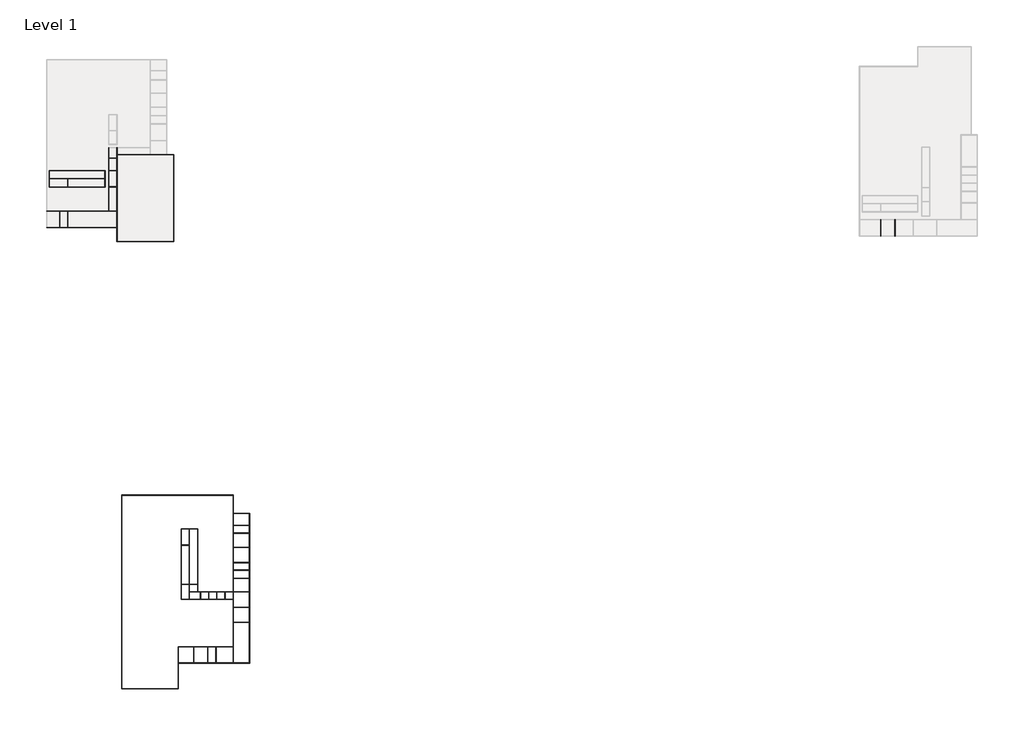
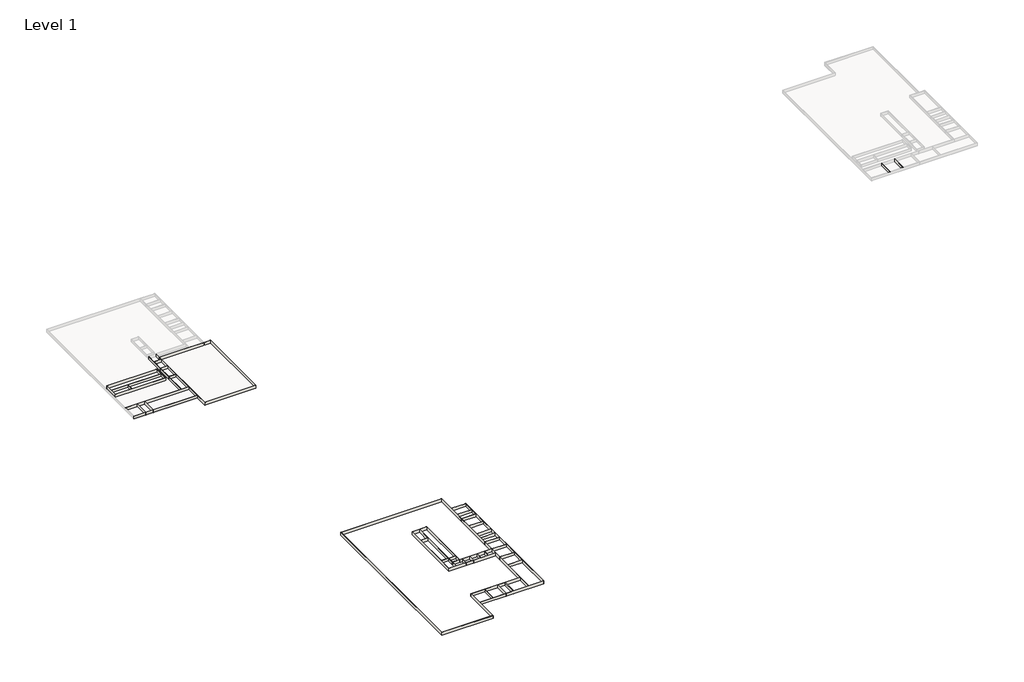
# One storey, part 1 of 4: 54 walls.
"""IFC4 building model written with IfcOpenShell, lengths in millimetres."""

from ifc_helpers import new_model, si_unit, origin, origin_with_axes, place, context, project, spatial, polyline, outline, extrude, faceted_brep, element, save

model = new_model("IFC4")

# Units and contexts
model_context = context("Model", 3, world=origin())
ifc_project = project(units=[si_unit("LENGTHUNIT", "METRE", prefix="MILLI")], contexts=[model_context])

# Site, building, storey
site = spatial("IfcSite", under=ifc_project)
building = spatial("IfcBuilding", under=site)
storey = spatial("IfcBuildingStorey", under=building, Name="Level 1", Elevation=0.0)

# Walls
placement = place(None, origin())
element("IfcWall", 1, ObjectType="Generic - 6\"", at=placement, inside=storey, context=model_context, shape_type="SweptSolid", body=[
    extrude(outline(polyline([(620688.6210536, -97824.0338454), (620688.6210536, -79688.4338454), (620841.0210536, -79688.4338454), (620841.0210536, -97824.0338454), (620688.6210536, -97824.0338454)])), origin_with_axes(), (0.0, 0.0, 1.0), 3657.6),
])
element("IfcWall", 2, ObjectType="Generic - 6\"", at=placement, inside=storey, context=model_context, shape_type="SweptSolid", body=[
    extrude(outline(polyline([(636538.2210536, -97824.0338454), (636538.2210536, -79688.4338454), (636690.6210536, -79688.4338454), (636690.6210536, -97824.0338454), (636538.2210536, -97824.0338454)])), origin_with_axes(), (0.0, 0.0, 1.0), 3657.6),
])
element("IfcWall", 3, ObjectType="Generic - 6\"", at=placement, inside=storey, context=model_context, shape_type="Brep", body=[
    faceted_brep([(-232744.5777071, -103934.3164234, 0.0), (-232744.5777071, -103781.9164234, 0.0), (-232744.5777071, -6780.7164234, 0.0), (-232744.5777071, -6628.3164234, 0.0), (-232744.5777071, 839.2835766, 0.0), (-232744.5777071, 839.2835766, 3657.6), (-232744.5777071, -6628.3164234, 3657.6), (-232744.5777071, -6780.7164234, 3657.6), (-232744.5777071, -103781.9164234, 3657.6), (-232744.5777071, -103934.3164234, 3657.6), (-232896.9777071, -103934.3164234, 0.0), (-232896.9777071, -103934.3164234, 3657.6), (-232896.9777071, -88376.6812497, 3657.6), (-232896.9777071, -88224.2812497, 3657.6), (-232896.9777071, -70088.6812497, 3657.6), (-232896.9777071, -69936.2812497, 3657.6), (-232896.9777071, -42899.5164234, 3657.6), (-232896.9777071, -42747.1164234, 3657.6), (-232896.9777071, -24763.9164234, 3657.6), (-232896.9777071, -24611.5164234, 3657.6), (-232896.9777071, -10895.5164234, 3657.6), (-232896.9777071, -10743.1164234, 3657.6), (-232896.9777071, 839.2835766, 3657.6), (-232896.9777071, 839.2835766, 0.0), (-232896.9777071, -10743.1164234, 0.0), (-232896.9777071, -10895.5164234, 0.0), (-232896.9777071, -24611.5164234, 0.0), (-232896.9777071, -24763.9164234, 0.0), (-232896.9777071, -42747.1164234, 0.0), (-232896.9777071, -42899.5164234, 0.0), (-232896.9777071, -69936.2812497, 0.0), (-232896.9777071, -70088.6812497, 0.0), (-232896.9777071, -88224.2812497, 0.0), (-232896.9777071, -88376.6812497, 0.0)], [[[0, 1, 2, 3, 4, 5, 6, 7, 8, 9]], [[10, 11, 12, 13, 14, 15, 16, 17, 18, 19, 20, 21, 22, 23, 24, 25, 26, 27, 28, 29, 30, 31, 32, 33]], [[4, 3, 2, 1, 0, 10, 33, 32, 31, 30, 29, 28, 27, 26, 25, 24, 23]], [[9, 8, 7, 6, 5, 22, 21, 20, 19, 18, 17, 16, 15, 14, 13, 12, 11]], [[0, 9, 11, 10]], [[5, 4, 23, 22]]]),
])
element("IfcWall", 4, ObjectType="Generic - 6\"", at=placement, inside=storey, context=model_context, shape_type="Brep", body=[
    faceted_brep([(-246155.7777071, -42899.5164234, 0.0), (-246308.1777071, -42899.5164234, 0.0), (-287608.5777071, -42899.5164234, 0.0), (-287760.9777071, -42899.5164234, 0.0), (-308258.7777071, -42899.5164234, 0.0), (-308411.1777071, -42899.5164234, 0.0), (-308411.1777071, -42899.5164234, 3657.6), (-308258.7777071, -42899.5164234, 3657.6), (-287760.9777071, -42899.5164234, 3657.6), (-287608.5777071, -42899.5164234, 3657.6), (-246308.1777071, -42899.5164234, 3657.6), (-246155.7777071, -42899.5164234, 3657.6), (-246155.7777071, -43051.9164234, 0.0), (-246155.7777071, -43051.9164234, 3657.6), (-308411.1777071, -43051.9164234, 3657.6), (-308411.1777071, -43051.9164234, 0.0)], [[[0, 1, 2, 3, 4, 5, 6, 7, 8, 9, 10, 11]], [[12, 13, 14, 15]], [[5, 4, 3, 2, 1, 0, 12, 15]], [[11, 10, 9, 8, 7, 6, 14, 13]], [[6, 5, 15, 14]], [[0, 11, 13, 12]]]),
])
element("IfcWall", 5, ObjectType="Generic - 6\"", at=placement, inside=storey, context=model_context, shape_type="SweptSolid", body=[
    extrude(outline(polyline([(-232896.9777071, -42899.5164234), (-241888.5777071, -42899.5164234), (-241888.5777071, -42747.1164234), (-232896.9777071, -42747.1164234), (-232896.9777071, -42899.5164234)])), origin_with_axes(), (0.0, 0.0, 1.0), 3657.6),
])
element("IfcWall", 6, ObjectType="Generic - 6\"", at=placement, inside=storey, context=model_context, shape_type="Brep", body=[
    faceted_brep([(-246308.1777071, -33755.5164234, 0.0), (-308258.7777071, -33755.5164234, 0.0), (-308258.7777071, -33755.5164234, 3657.6), (-246308.1777071, -33755.5164234, 3657.6), (-246308.1777071, -33907.9164234, 0.0), (-246308.1777071, -33907.9164234, 3657.6), (-287608.5777071, -33907.9164234, 3657.6), (-287760.9777071, -33907.9164234, 3657.6), (-308258.7777071, -33907.9164234, 3657.6), (-308258.7777071, -33907.9164234, 0.0), (-287760.9777071, -33907.9164234, 0.0), (-287608.5777071, -33907.9164234, 0.0)], [[[0, 1, 2, 3]], [[4, 5, 6, 7, 8, 9, 10, 11]], [[1, 0, 4, 11, 10, 9]], [[3, 2, 8, 7, 6, 5]], [[2, 1, 9, 8]], [[0, 3, 5, 4]]]),
])
element("IfcWall", 7, ObjectType="Generic - 6\"", at=placement, inside=storey, context=model_context, shape_type="Brep", body=[
    faceted_brep([(-246155.7777071, -24611.5164234, 0.0), (-308411.1777071, -24611.5164234, 0.0), (-308411.1777071, -24611.5164234, 3657.6), (-246155.7777071, -24611.5164234, 3657.6), (-246155.7777071, -24763.9164234, 0.0), (-246155.7777071, -24763.9164234, 3657.6), (-246308.1777071, -24763.9164234, 3657.6), (-308258.7777071, -24763.9164234, 3657.6), (-308411.1777071, -24763.9164234, 3657.6), (-308411.1777071, -24763.9164234, 0.0), (-308258.7777071, -24763.9164234, 0.0), (-246308.1777071, -24763.9164234, 0.0)], [[[0, 1, 2, 3]], [[4, 5, 6, 7, 8, 9, 10, 11]], [[1, 0, 4, 11, 10, 9]], [[3, 2, 8, 7, 6, 5]], [[2, 1, 9, 8]], [[0, 3, 5, 4]]]),
])
element("IfcWall", 8, ObjectType="Generic - 6\"", at=placement, inside=storey, context=model_context, shape_type="Brep", body=[
    faceted_brep([(-169189.5777071, -6628.3164234, 0.0), (-177212.1746874, -6628.3164234, 0.0), (-177364.5746874, -6628.3164234, 0.0), (-195500.1746874, -6628.3164234, 0.0), (-195652.5746874, -6628.3164234, 0.0), (-232744.5777071, -6628.3164234, 0.0), (-232744.5777071, -6628.3164234, 3657.6), (-195652.5746874, -6628.3164234, 3657.6), (-195500.1746874, -6628.3164234, 3657.6), (-177364.5746874, -6628.3164234, 3657.6), (-177212.1746874, -6628.3164234, 3657.6), (-169189.5777071, -6628.3164234, 3657.6), (-169189.5777071, -6780.7164234, 0.0), (-169189.5777071, -6780.7164234, 3657.6), (-169341.9777071, -6780.7164234, 3657.6), (-232744.5777071, -6780.7164234, 3657.6), (-232744.5777071, -6780.7164234, 0.0), (-169341.9777071, -6780.7164234, 0.0)], [[[0, 1, 2, 3, 4, 5, 6, 7, 8, 9, 10, 11]], [[12, 13, 14, 15, 16, 17]], [[5, 4, 3, 2, 1, 0, 12, 17, 16]], [[11, 10, 9, 8, 7, 6, 15, 14, 13]], [[0, 11, 13, 12]], [[6, 5, 16, 15]]]),
])
element("IfcWall", 9, ObjectType="Generic - 6\"", at=placement, inside=storey, context=model_context, shape_type="Brep", body=[
    faceted_brep([(-308411.1777071, -24763.9164234, 0.0), (-308411.1777071, -42899.5164234, 0.0), (-308411.1777071, -42899.5164234, 3657.6), (-308411.1777071, -24763.9164234, 3657.6), (-308258.7777071, -24763.9164234, 0.0), (-308258.7777071, -24763.9164234, 3657.6), (-308258.7777071, -33755.5164234, 3657.6), (-308258.7777071, -33907.9164234, 3657.6), (-308258.7777071, -42899.5164234, 3657.6), (-308258.7777071, -42899.5164234, 0.0), (-308258.7777071, -33907.9164234, 0.0), (-308258.7777071, -33755.5164234, 0.0)], [[[0, 1, 2, 3]], [[4, 5, 6, 7, 8, 9, 10, 11]], [[1, 0, 4, 11, 10, 9]], [[3, 2, 8, 7, 6, 5]], [[0, 3, 5, 4]], [[2, 1, 9, 8]]]),
])
element("IfcWall", 10, ObjectType="Generic - 6\"", at=placement, inside=storey, context=model_context, shape_type="SweptSolid", body=[
    extrude(outline(polyline([(-287760.9777071, -42899.5164234), (-287760.9777071, -33907.9164234), (-287608.5777071, -33907.9164234), (-287608.5777071, -42899.5164234), (-287760.9777071, -42899.5164234)])), origin_with_axes(), (0.0, 0.0, 1.0), 3657.6),
])
element("IfcWall", 11, ObjectType="Generic - 6\"", at=placement, inside=storey, context=model_context, shape_type="Brep", body=[
    faceted_brep([(-232896.9777071, -88224.2812497, 0.0), (-287608.5777071, -88224.2812497, 0.0), (-287760.9777071, -88224.2812497, 0.0), (-296752.5777071, -88224.2812497, 0.0), (-296904.9777071, -88224.2812497, 0.0), (-311382.9777071, -88224.2812497, 0.0), (-311535.3777071, -88224.2812497, 0.0), (-311535.3777071, -88224.2812497, 3657.6), (-311382.9777071, -88224.2812497, 3657.6), (-296904.9777071, -88224.2812497, 3657.6), (-296752.5777071, -88224.2812497, 3657.6), (-287760.9777071, -88224.2812497, 3657.6), (-287608.5777071, -88224.2812497, 3657.6), (-232896.9777071, -88224.2812497, 3657.6), (-232896.9777071, -88376.6812497, 0.0), (-232896.9777071, -88376.6812497, 3657.6), (-311535.3777071, -88376.6812497, 3657.6), (-311535.3777071, -88376.6812497, 0.0)], [[[0, 1, 2, 3, 4, 5, 6, 7, 8, 9, 10, 11, 12, 13]], [[14, 15, 16, 17]], [[6, 5, 4, 3, 2, 1, 0, 14, 17]], [[13, 12, 11, 10, 9, 8, 7, 16, 15]], [[7, 6, 17, 16]], [[0, 13, 15, 14]]]),
])
element("IfcWall", 12, ObjectType="Generic - 6\"", at=placement, inside=storey, context=model_context, shape_type="Brep", body=[
    faceted_brep([(-232896.9777071, -69936.2812497, 0.0), (-241888.5777071, -69936.2812497, 0.0), (-242040.9777071, -69936.2812497, 0.0), (-311382.9777071, -69936.2812497, 0.0), (-311382.9777071, -69936.2812497, 3657.6), (-242040.9777071, -69936.2812497, 3657.6), (-241888.5777071, -69936.2812497, 3657.6), (-232896.9777071, -69936.2812497, 3657.6), (-232896.9777071, -70088.6812497, 0.0), (-232896.9777071, -70088.6812497, 3657.6), (-287608.5777071, -70088.6812497, 3657.6), (-287760.9777071, -70088.6812497, 3657.6), (-296752.5777071, -70088.6812497, 3657.6), (-296904.9777071, -70088.6812497, 3657.6), (-311382.9777071, -70088.6812497, 3657.6), (-311382.9777071, -70088.6812497, 0.0), (-296904.9777071, -70088.6812497, 0.0), (-296752.5777071, -70088.6812497, 0.0), (-287760.9777071, -70088.6812497, 0.0), (-287608.5777071, -70088.6812497, 0.0)], [[[0, 1, 2, 3, 4, 5, 6, 7]], [[8, 9, 10, 11, 12, 13, 14, 15, 16, 17, 18, 19]], [[3, 2, 1, 0, 8, 19, 18, 17, 16, 15]], [[7, 6, 5, 4, 14, 13, 12, 11, 10, 9]], [[0, 7, 9, 8]], [[4, 3, 15, 14]]]),
])
element("IfcWall", 13, ObjectType="Generic - 6\"", at=placement, inside=storey, context=model_context, shape_type="SweptSolid", body=[
    extrude(outline(polyline([(-287760.9777071, -88224.2812497), (-287760.9777071, -70088.6812497), (-287608.5777071, -70088.6812497), (-287608.5777071, -88224.2812497), (-287760.9777071, -88224.2812497)])), origin_with_axes(), (0.0, 0.0, 1.0), 3657.6),
])
element("IfcWall", 14, ObjectType="Generic - 6\"", at=placement, inside=storey, context=model_context, shape_type="SweptSolid", body=[
    extrude(outline(polyline([(-296904.9777071, -88224.2812497), (-296904.9777071, -70088.6812497), (-296752.5777071, -70088.6812497), (-296752.5777071, -88224.2812497), (-296904.9777071, -88224.2812497)])), origin_with_axes(), (0.0, 0.0, 1.0), 3657.6),
])
element("IfcWall", 15, ObjectType="Generic - 6\"", at=placement, inside=storey, context=model_context, shape_type="Brep", body=[
    faceted_brep([(-169341.9777071, -6780.7164234, 0.0), (-169341.9777071, -103781.9164234, 0.0), (-169341.9777071, -103934.3164234, 0.0), (-169341.9777071, -103934.3164234, 3657.6), (-169341.9777071, -103781.9164234, 3657.6), (-169341.9777071, -6780.7164234, 3657.6), (-169189.5777071, -6780.7164234, 0.0), (-169189.5777071, -6780.7164234, 3657.6), (-169189.5777071, -103934.3164234, 3657.6), (-169189.5777071, -103934.3164234, 0.0)], [[[0, 1, 2, 3, 4, 5]], [[6, 7, 8, 9]], [[2, 1, 0, 6, 9]], [[5, 4, 3, 8, 7]], [[3, 2, 9, 8]], [[0, 5, 7, 6]]]),
])
element("IfcWall", 16, ObjectType="Generic - 6\"", at=placement, inside=storey, context=model_context, shape_type="SweptSolid", body=[
    extrude(outline(polyline([(-232744.5777071, -103781.9164234), (-169341.9777071, -103781.9164234), (-169341.9777071, -103934.3164234), (-232744.5777071, -103934.3164234), (-232744.5777071, -103781.9164234)])), origin_with_axes(), (0.0, 0.0, 1.0), 3657.6),
])
element("IfcWall", 17, ObjectType="Generic - 6\"", at=placement, inside=storey, context=model_context, shape_type="SweptSolid", body=[
    extrude(outline(polyline([(-241888.5777071, -24611.5164234), (-232896.9777071, -24611.5164234), (-232896.9777071, -24763.9164234), (-241888.5777071, -24763.9164234), (-241888.5777071, -24611.5164234)])), origin_with_axes(), (0.0, 0.0, 1.0), 3657.6),
])
element("IfcWall", 18, ObjectType="Generic - 6\"", at=placement, inside=storey, context=model_context, shape_type="Brep", body=[
    faceted_brep([(-246308.1777071, -24763.9164234, 0.0), (-246308.1777071, -33755.5164234, 0.0), (-246308.1777071, -33907.9164234, 0.0), (-246308.1777071, -42899.5164234, 0.0), (-246308.1777071, -42899.5164234, 3657.6), (-246308.1777071, -33907.9164234, 3657.6), (-246308.1777071, -33755.5164234, 3657.6), (-246308.1777071, -24763.9164234, 3657.6), (-246155.7777071, -24763.9164234, 0.0), (-246155.7777071, -24763.9164234, 3657.6), (-246155.7777071, -42899.5164234, 3657.6), (-246155.7777071, -42899.5164234, 0.0)], [[[0, 1, 2, 3, 4, 5, 6, 7]], [[8, 9, 10, 11]], [[3, 2, 1, 0, 8, 11]], [[7, 6, 5, 4, 10, 9]], [[4, 3, 11, 10]], [[0, 7, 9, 8]]]),
])
element("IfcWall", 19, ObjectType="Generic - 6\"", at=placement, inside=storey, context=model_context, shape_type="Brep", body=[
    faceted_brep([(-242040.9777071, 839.2835766, 0.0), (-242040.9777071, -69936.2812497, 0.0), (-242040.9777071, -69936.2812497, 3657.6), (-242040.9777071, 839.2835766, 3657.6), (-241888.5777071, 839.2835766, 0.0), (-241888.5777071, 839.2835766, 3657.6), (-241888.5777071, -10743.1164234, 3657.6), (-241888.5777071, -10895.5164234, 3657.6), (-241888.5777071, -24611.5164234, 3657.6), (-241888.5777071, -24763.9164234, 3657.6), (-241888.5777071, -42747.1164234, 3657.6), (-241888.5777071, -42899.5164234, 3657.6), (-241888.5777071, -69936.2812497, 3657.6), (-241888.5777071, -69936.2812497, 0.0), (-241888.5777071, -42899.5164234, 0.0), (-241888.5777071, -42747.1164234, 0.0), (-241888.5777071, -24763.9164234, 0.0), (-241888.5777071, -24611.5164234, 0.0), (-241888.5777071, -10895.5164234, 0.0), (-241888.5777071, -10743.1164234, 0.0)], [[[0, 1, 2, 3]], [[4, 5, 6, 7, 8, 9, 10, 11, 12, 13, 14, 15, 16, 17, 18, 19]], [[1, 0, 4, 19, 18, 17, 16, 15, 14, 13]], [[3, 2, 12, 11, 10, 9, 8, 7, 6, 5]], [[2, 1, 13, 12]], [[0, 3, 5, 4]]]),
])
element("IfcWall", 20, ObjectType="Generic - 6\"", at=placement, inside=storey, context=model_context, shape_type="SweptSolid", body=[
    extrude(outline(polyline([(-241888.5777071, -10743.1164234), (-232896.9777071, -10743.1164234), (-232896.9777071, -10895.5164234), (-241888.5777071, -10895.5164234), (-241888.5777071, -10743.1164234)])), origin_with_axes(), (0.0, 0.0, 1.0), 3657.6),
])
element("IfcWall", 21, ObjectType="Generic - 6\"", at=placement, inside=storey, context=model_context, shape_type="SweptSolid", body=[
    extrude(outline(polyline([(-84744.5931462, -408234.2669954), (-102880.1931462, -408234.2669954), (-102880.1931462, -408081.8669954), (-84744.5931462, -408081.8669954), (-84744.5931462, -408234.2669954)])), origin_with_axes(), (0.0, 0.0, 1.0), 3657.6),
])
element("IfcWall", 22, ObjectType="Generic - 6\"", at=placement, inside=storey, context=model_context, shape_type="Brep", body=[
    faceted_brep([(-102880.1931462, -575355.6713404, 0.0), (-102880.1931462, -529788.0713404, 0.0), (-102880.1931462, -529635.6713404, 0.0), (-102880.1931462, -513085.4669954, 0.0), (-102880.1931462, -512933.0669954, 0.0), (-102880.1931462, -495822.6381278, 0.0), (-102880.1931462, -495670.2381278, 0.0), (-102880.1931462, -480776.6669954, 0.0), (-102880.1931462, -480624.2669954, 0.0), (-102880.1931462, -471480.2669954, 0.0), (-102880.1931462, -471327.8669954, 0.0), (-102880.1931462, -463098.2669954, 0.0), (-102880.1931462, -462945.8669954, 0.0), (-102880.1931462, -446029.4669954, 0.0), (-102880.1931462, -445877.0669954, 0.0), (-102880.1931462, -430179.8669954, 0.0), (-102880.1931462, -430027.4669954, 0.0), (-102880.1931462, -421340.6669954, 0.0), (-102880.1931462, -421188.2669954, 0.0), (-102880.1931462, -408234.2669954, 0.0), (-102880.1931462, -408081.8669954, 0.0), (-102880.1931462, -387751.2713404, 0.0), (-102880.1931462, -387751.2713404, 3657.6), (-102880.1931462, -408081.8669954, 3657.6), (-102880.1931462, -408234.2669954, 3657.6), (-102880.1931462, -421188.2669954, 3657.6), (-102880.1931462, -421340.6669954, 3657.6), (-102880.1931462, -430027.4669954, 3657.6), (-102880.1931462, -430179.8669954, 3657.6), (-102880.1931462, -445877.0669954, 3657.6), (-102880.1931462, -446029.4669954, 3657.6), (-102880.1931462, -462945.8669954, 3657.6), (-102880.1931462, -463098.2669954, 3657.6), (-102880.1931462, -471327.8669954, 3657.6), (-102880.1931462, -471480.2669954, 3657.6), (-102880.1931462, -480624.2669954, 3657.6), (-102880.1931462, -480776.6669954, 3657.6), (-102880.1931462, -495670.2381278, 3657.6), (-102880.1931462, -495822.6381278, 3657.6), (-102880.1931462, -512933.0669954, 3657.6), (-102880.1931462, -513085.4669954, 3657.6), (-102880.1931462, -529635.6713404, 3657.6), (-102880.1931462, -529788.0713404, 3657.6), (-102880.1931462, -575355.6713404, 3657.6), (-103032.5931462, -575355.6713404, 0.0), (-103032.5931462, -575355.6713404, 3657.6), (-103032.5931462, -557220.0713404, 3657.6), (-103032.5931462, -557067.6713404, 3657.6), (-103032.5931462, -504239.2092603, 3657.6), (-103032.5931462, -504086.8092603, 3657.6), (-103032.5931462, -495822.6381278, 3657.6), (-103032.5931462, -495670.2381278, 3657.6), (-103032.5931462, -387751.2713404, 3657.6), (-103032.5931462, -387751.2713404, 0.0), (-103032.5931462, -495670.2381278, 0.0), (-103032.5931462, -495822.6381278, 0.0), (-103032.5931462, -504086.8092603, 0.0), (-103032.5931462, -504239.2092603, 0.0), (-103032.5931462, -557067.6713404, 0.0), (-103032.5931462, -557220.0713404, 0.0)], [[[0, 1, 2, 3, 4, 5, 6, 7, 8, 9, 10, 11, 12, 13, 14, 15, 16, 17, 18, 19, 20, 21, 22, 23, 24, 25, 26, 27, 28, 29, 30, 31, 32, 33, 34, 35, 36, 37, 38, 39, 40, 41, 42, 43]], [[44, 45, 46, 47, 48, 49, 50, 51, 52, 53, 54, 55, 56, 57, 58, 59]], [[21, 20, 19, 18, 17, 16, 15, 14, 13, 12, 11, 10, 9, 8, 7, 6, 5, 4, 3, 2, 1, 0, 44, 59, 58, 57, 56, 55, 54, 53]], [[43, 42, 41, 40, 39, 38, 37, 36, 35, 34, 33, 32, 31, 30, 29, 28, 27, 26, 25, 24, 23, 22, 52, 51, 50, 49, 48, 47, 46, 45]], [[22, 21, 53, 52]], [[0, 43, 45, 44]]]),
])
element("IfcWall", 23, ObjectType="Generic - 6\"", at=placement, inside=storey, context=model_context, shape_type="Brep", body=[
    faceted_brep([(-84744.5931462, -408081.8669954, 0.0), (-84744.5931462, -408234.2669954, 0.0), (-84744.5931462, -421188.2669954, 0.0), (-84744.5931462, -421340.6669954, 0.0), (-84744.5931462, -430027.4669954, 0.0), (-84744.5931462, -430179.8669954, 0.0), (-84744.5931462, -445877.0669954, 0.0), (-84744.5931462, -446029.4669954, 0.0), (-84744.5931462, -462945.8669954, 0.0), (-84744.5931462, -463098.2669954, 0.0), (-84744.5931462, -471327.8669954, 0.0), (-84744.5931462, -471480.2669954, 0.0), (-84744.5931462, -480624.2669954, 0.0), (-84744.5931462, -480776.6669954, 0.0), (-84744.5931462, -495670.2381278, 0.0), (-84744.5931462, -495822.6381278, 0.0), (-84744.5931462, -512933.0669954, 0.0), (-84744.5931462, -513085.4669954, 0.0), (-84744.5931462, -529635.6713404, 0.0), (-84744.5931462, -529788.0713404, 0.0), (-84744.5931462, -575355.6713404, 0.0), (-84744.5931462, -575508.0713404, 0.0), (-84744.5931462, -575508.0713404, 3657.6), (-84744.5931462, -575355.6713404, 3657.6), (-84744.5931462, -529788.0713404, 3657.6), (-84744.5931462, -529635.6713404, 3657.6), (-84744.5931462, -513085.4669954, 3657.6), (-84744.5931462, -512933.0669954, 3657.6), (-84744.5931462, -495822.6381278, 3657.6), (-84744.5931462, -495670.2381278, 3657.6), (-84744.5931462, -480776.6669954, 3657.6), (-84744.5931462, -480624.2669954, 3657.6), (-84744.5931462, -471480.2669954, 3657.6), (-84744.5931462, -471327.8669954, 3657.6), (-84744.5931462, -463098.2669954, 3657.6), (-84744.5931462, -462945.8669954, 3657.6), (-84744.5931462, -446029.4669954, 3657.6), (-84744.5931462, -445877.0669954, 3657.6), (-84744.5931462, -430179.8669954, 3657.6), (-84744.5931462, -430027.4669954, 3657.6), (-84744.5931462, -421340.6669954, 3657.6), (-84744.5931462, -421188.2669954, 3657.6), (-84744.5931462, -408234.2669954, 3657.6), (-84744.5931462, -408081.8669954, 3657.6), (-84592.1931462, -408081.8669954, 0.0), (-84592.1931462, -408081.8669954, 3657.6), (-84592.1931462, -575508.0713404, 3657.6), (-84592.1931462, -575508.0713404, 0.0)], [[[0, 1, 2, 3, 4, 5, 6, 7, 8, 9, 10, 11, 12, 13, 14, 15, 16, 17, 18, 19, 20, 21, 22, 23, 24, 25, 26, 27, 28, 29, 30, 31, 32, 33, 34, 35, 36, 37, 38, 39, 40, 41, 42, 43]], [[44, 45, 46, 47]], [[21, 20, 19, 18, 17, 16, 15, 14, 13, 12, 11, 10, 9, 8, 7, 6, 5, 4, 3, 2, 1, 0, 44, 47]], [[43, 42, 41, 40, 39, 38, 37, 36, 35, 34, 33, 32, 31, 30, 29, 28, 27, 26, 25, 24, 23, 22, 46, 45]], [[0, 43, 45, 44]], [[22, 21, 47, 46]]]),
])
element("IfcWall", 24, ObjectType="Generic - 6\"", at=placement, inside=storey, context=model_context, shape_type="Brep", body=[
    faceted_brep([(-164230.6008654, -557220.0713404, 0.0), (-164078.2008654, -557220.0713404, 0.0), (-147161.8008654, -557220.0713404, 0.0), (-147009.4008654, -557220.0713404, 0.0), (-131312.2008654, -557220.0713404, 0.0), (-131159.8008654, -557220.0713404, 0.0), (-122168.2008654, -557220.0713404, 0.0), (-122015.8008654, -557220.0713404, 0.0), (-103032.5931462, -557220.0713404, 0.0), (-103032.5931462, -557220.0713404, 3657.6), (-122015.8008654, -557220.0713404, 3657.6), (-122168.2008654, -557220.0713404, 3657.6), (-131159.8008654, -557220.0713404, 3657.6), (-131312.2008654, -557220.0713404, 3657.6), (-147009.4008654, -557220.0713404, 3657.6), (-147161.8008654, -557220.0713404, 3657.6), (-164078.2008654, -557220.0713404, 3657.6), (-164230.6008654, -557220.0713404, 3657.6), (-164230.6008654, -557067.6713404, 0.0), (-164230.6008654, -557067.6713404, 3657.6), (-103032.5931462, -557067.6713404, 3657.6), (-103032.5931462, -557067.6713404, 0.0)], [[[0, 1, 2, 3, 4, 5, 6, 7, 8, 9, 10, 11, 12, 13, 14, 15, 16, 17]], [[18, 19, 20, 21]], [[8, 7, 6, 5, 4, 3, 2, 1, 0, 18, 21]], [[17, 16, 15, 14, 13, 12, 11, 10, 9, 20, 19]], [[0, 17, 19, 18]], [[9, 8, 21, 20]]]),
])
element("IfcWall", 25, ObjectType="Generic - 6\"", at=placement, inside=storey, context=model_context, shape_type="Brep", body=[
    faceted_brep([(-164078.2008654, -604385.7770193, 0.0), (-164078.2008654, -575508.0713404, 0.0), (-164078.2008654, -575355.6713404, 0.0), (-164078.2008654, -557220.0713404, 0.0), (-164078.2008654, -557220.0713404, 3657.6), (-164078.2008654, -575355.6713404, 3657.6), (-164078.2008654, -575508.0713404, 3657.6), (-164078.2008654, -604385.7770193, 3657.6), (-164230.6008654, -604385.7770193, 0.0), (-164230.6008654, -604385.7770193, 3657.6), (-164230.6008654, -604233.3770193, 3657.6), (-164230.6008654, -557220.0713404, 3657.6), (-164230.6008654, -557220.0713404, 0.0), (-164230.6008654, -604233.3770193, 0.0)], [[[0, 1, 2, 3, 4, 5, 6, 7]], [[8, 9, 10, 11, 12, 13]], [[3, 2, 1, 0, 8, 13, 12]], [[7, 6, 5, 4, 11, 10, 9]], [[4, 3, 12, 11]], [[0, 7, 9, 8]]]),
])
element("IfcWall", 26, ObjectType="Generic - 6\"", at=placement, inside=storey, context=model_context, shape_type="Brep", body=[
    faceted_brep([(-84744.5931462, -575355.6713404, 0.0), (-102880.1931462, -575355.6713404, 0.0), (-103032.5931462, -575355.6713404, 0.0), (-122015.8008654, -575355.6713404, 0.0), (-122168.2008654, -575355.6713404, 0.0), (-131159.8008654, -575355.6713404, 0.0), (-131312.2008654, -575355.6713404, 0.0), (-147009.4008654, -575355.6713404, 0.0), (-147161.8008654, -575355.6713404, 0.0), (-164078.2008654, -575355.6713404, 0.0), (-164078.2008654, -575355.6713404, 3657.6), (-147161.8008654, -575355.6713404, 3657.6), (-147009.4008654, -575355.6713404, 3657.6), (-131312.2008654, -575355.6713404, 3657.6), (-131159.8008654, -575355.6713404, 3657.6), (-122168.2008654, -575355.6713404, 3657.6), (-122015.8008654, -575355.6713404, 3657.6), (-103032.5931462, -575355.6713404, 3657.6), (-102880.1931462, -575355.6713404, 3657.6), (-84744.5931462, -575355.6713404, 3657.6), (-84744.5931462, -575508.0713404, 0.0), (-84744.5931462, -575508.0713404, 3657.6), (-164078.2008654, -575508.0713404, 3657.6), (-164078.2008654, -575508.0713404, 0.0)], [[[0, 1, 2, 3, 4, 5, 6, 7, 8, 9, 10, 11, 12, 13, 14, 15, 16, 17, 18, 19]], [[20, 21, 22, 23]], [[9, 8, 7, 6, 5, 4, 3, 2, 1, 0, 20, 23]], [[19, 18, 17, 16, 15, 14, 13, 12, 11, 10, 22, 21]], [[0, 19, 21, 20]], [[10, 9, 23, 22]]]),
])
element("IfcWall", 27, ObjectType="Generic - 6\"", at=placement, inside=storey, context=model_context, shape_type="Brep", body=[
    faceted_brep([(-164230.6008654, -604233.3770193, 0.0), (-227512.7956392, -604233.3770193, 0.0), (-227665.1956392, -604233.3770193, 0.0), (-227665.1956392, -604233.3770193, 3657.6), (-227512.7956392, -604233.3770193, 3657.6), (-164230.6008654, -604233.3770193, 3657.6), (-164230.6008654, -604385.7770193, 0.0), (-164230.6008654, -604385.7770193, 3657.6), (-227665.1956392, -604385.7770193, 3657.6), (-227665.1956392, -604385.7770193, 0.0)], [[[0, 1, 2, 3, 4, 5]], [[6, 7, 8, 9]], [[2, 1, 0, 6, 9]], [[5, 4, 3, 8, 7]], [[0, 5, 7, 6]], [[3, 2, 9, 8]]]),
])
element("IfcWall", 28, ObjectType="Generic - 6\"", at=placement, inside=storey, context=model_context, shape_type="Brep", body=[
    faceted_brep([(-227512.7956392, -604233.3770193, 0.0), (-227512.7956392, -387751.2713404, 0.0), (-227512.7956392, -387598.8713404, 0.0), (-227512.7956392, -387598.8713404, 3657.6), (-227512.7956392, -387751.2713404, 3657.6), (-227512.7956392, -604233.3770193, 3657.6), (-227665.1956392, -604233.3770193, 0.0), (-227665.1956392, -604233.3770193, 3657.6), (-227665.1956392, -387598.8713404, 3657.6), (-227665.1956392, -387598.8713404, 0.0)], [[[0, 1, 2, 3, 4, 5]], [[6, 7, 8, 9]], [[2, 1, 0, 6, 9]], [[5, 4, 3, 8, 7]], [[0, 5, 7, 6]], [[3, 2, 9, 8]]]),
])
element("IfcWall", 29, ObjectType="Generic - 6\"", at=placement, inside=storey, context=model_context, shape_type="Brep", body=[
    faceted_brep([(-227512.7956392, -387751.2713404, 0.0), (-103032.5931462, -387751.2713404, 0.0), (-102880.1931462, -387751.2713404, 0.0), (-102880.1931462, -387751.2713404, 3657.6), (-103032.5931462, -387751.2713404, 3657.6), (-227512.7956392, -387751.2713404, 3657.6), (-227512.7956392, -387598.8713404, 0.0), (-227512.7956392, -387598.8713404, 3657.6), (-102880.1931462, -387598.8713404, 3657.6), (-102880.1931462, -387598.8713404, 0.0)], [[[0, 1, 2, 3, 4, 5]], [[6, 7, 8, 9]], [[2, 1, 0, 6, 9]], [[5, 4, 3, 8, 7]], [[0, 5, 7, 6]], [[3, 2, 9, 8]]]),
])
element("IfcWall", 30, ObjectType="Generic - 6\"", at=placement, inside=storey, context=model_context, shape_type="SweptSolid", body=[
    extrude(outline(polyline([(-84744.5931462, -421340.6669954), (-102880.1931462, -421340.6669954), (-102880.1931462, -421188.2669954), (-84744.5931462, -421188.2669954), (-84744.5931462, -421340.6669954)])), origin_with_axes(), (0.0, 0.0, 1.0), 3657.6),
])
element("IfcWall", 31, ObjectType="Generic - 6\"", at=placement, inside=storey, context=model_context, shape_type="SweptSolid", body=[
    extrude(outline(polyline([(-84744.5931462, -446029.4669954), (-102880.1931462, -446029.4669954), (-102880.1931462, -445877.0669954), (-84744.5931462, -445877.0669954), (-84744.5931462, -446029.4669954)])), origin_with_axes(), (0.0, 0.0, 1.0), 3657.6),
])
element("IfcWall", 32, ObjectType="Generic - 6\"", at=placement, inside=storey, context=model_context, shape_type="SweptSolid", body=[
    extrude(outline(polyline([(-84744.5931462, -463098.2669954), (-102880.1931462, -463098.2669954), (-102880.1931462, -462945.8669954), (-84744.5931462, -462945.8669954), (-84744.5931462, -463098.2669954)])), origin_with_axes(), (0.0, 0.0, 1.0), 3657.6),
])
element("IfcWall", 33, ObjectType="Generic - 6\"", at=placement, inside=storey, context=model_context, shape_type="SweptSolid", body=[
    extrude(outline(polyline([(-84744.5931462, -480776.6669954), (-102880.1931462, -480776.6669954), (-102880.1931462, -480624.2669954), (-84744.5931462, -480624.2669954), (-84744.5931462, -480776.6669954)])), origin_with_axes(), (0.0, 0.0, 1.0), 3657.6),
])
element("IfcWall", 34, ObjectType="Generic - 6\"", at=placement, inside=storey, context=model_context, shape_type="SweptSolid", body=[
    extrude(outline(polyline([(-84744.5931462, -495822.6381278), (-102880.1931462, -495822.6381278), (-102880.1931462, -495670.2381278), (-84744.5931462, -495670.2381278), (-84744.5931462, -495822.6381278)])), origin_with_axes(), (0.0, 0.0, 1.0), 3657.6),
])
element("IfcWall", 35, ObjectType="Generic - 6\"", at=placement, inside=storey, context=model_context, shape_type="SweptSolid", body=[
    extrude(outline(polyline([(-84744.5931462, -529788.0713404), (-102880.1931462, -529788.0713404), (-102880.1931462, -529635.6713404), (-84744.5931462, -529635.6713404), (-84744.5931462, -529788.0713404)])), origin_with_axes(), (0.0, 0.0, 1.0), 3657.6),
])
element("IfcWall", 36, ObjectType="Generic - 6\"", at=placement, inside=storey, context=model_context, shape_type="SweptSolid", body=[
    extrude(outline(polyline([(-147161.8008654, -575355.6713404), (-147161.8008654, -557220.0713404), (-147009.4008654, -557220.0713404), (-147009.4008654, -575355.6713404), (-147161.8008654, -575355.6713404)])), origin_with_axes(), (0.0, 0.0, 1.0), 3657.6),
])
element("IfcWall", 37, ObjectType="Generic - 6\"", at=placement, inside=storey, context=model_context, shape_type="SweptSolid", body=[
    extrude(outline(polyline([(-131312.2008654, -575355.6713404), (-131312.2008654, -557220.0713404), (-131159.8008654, -557220.0713404), (-131159.8008654, -575355.6713404), (-131312.2008654, -575355.6713404)])), origin_with_axes(), (0.0, 0.0, 1.0), 3657.6),
])
element("IfcWall", 38, ObjectType="Generic - 6\"", at=placement, inside=storey, context=model_context, shape_type="SweptSolid", body=[
    extrude(outline(polyline([(-122168.2008654, -575355.6713404), (-122168.2008654, -557220.0713404), (-122015.8008654, -557220.0713404), (-122015.8008654, -575355.6713404), (-122168.2008654, -575355.6713404)])), origin_with_axes(), (0.0, 0.0, 1.0), 3657.6),
])
element("IfcWall", 39, ObjectType="Generic - 6\"", at=placement, inside=storey, context=model_context, shape_type="Brep", body=[
    faceted_brep([(-160944.5931462, -504086.8092603, 0.0), (-160944.5931462, -487406.0669954, 0.0), (-160944.5931462, -487253.6669954, 0.0), (-160944.5931462, -443591.0669954, 0.0), (-160944.5931462, -443438.6669954, 0.0), (-160944.5931462, -425303.0669954, 0.0), (-160944.5931462, -425150.6669954, 0.0), (-160944.5931462, -425150.6669954, 3657.6), (-160944.5931462, -425303.0669954, 3657.6), (-160944.5931462, -443438.6669954, 3657.6), (-160944.5931462, -443591.0669954, 3657.6), (-160944.5931462, -487253.6669954, 3657.6), (-160944.5931462, -487406.0669954, 3657.6), (-160944.5931462, -504086.8092603, 3657.6), (-161096.9931462, -504086.8092603, 0.0), (-161096.9931462, -504086.8092603, 3657.6), (-161096.9931462, -425150.6669954, 3657.6), (-161096.9931462, -425150.6669954, 0.0)], [[[0, 1, 2, 3, 4, 5, 6, 7, 8, 9, 10, 11, 12, 13]], [[14, 15, 16, 17]], [[6, 5, 4, 3, 2, 1, 0, 14, 17]], [[13, 12, 11, 10, 9, 8, 7, 16, 15]], [[7, 6, 17, 16]], [[0, 13, 15, 14]]]),
])
element("IfcWall", 40, ObjectType="Generic - 6\"", at=placement, inside=storey, context=model_context, shape_type="Brep", body=[
    faceted_brep([(-142656.5931462, -495670.2381278, 0.0), (-142656.5931462, -425150.6669954, 0.0), (-142656.5931462, -425150.6669954, 3657.6), (-142656.5931462, -495670.2381278, 3657.6), (-142808.9931462, -495670.2381278, 0.0), (-142808.9931462, -495670.2381278, 3657.6), (-142808.9931462, -487406.0669954, 3657.6), (-142808.9931462, -487253.6669954, 3657.6), (-142808.9931462, -425303.0669954, 3657.6), (-142808.9931462, -425150.6669954, 3657.6), (-142808.9931462, -425150.6669954, 0.0), (-142808.9931462, -425303.0669954, 0.0), (-142808.9931462, -487253.6669954, 0.0), (-142808.9931462, -487406.0669954, 0.0)], [[[0, 1, 2, 3]], [[4, 5, 6, 7, 8, 9, 10, 11, 12, 13]], [[1, 0, 4, 13, 12, 11, 10]], [[3, 2, 9, 8, 7, 6, 5]], [[2, 1, 10, 9]], [[0, 3, 5, 4]]]),
])
element("IfcWall", 41, ObjectType="Generic - 6\"", at=placement, inside=storey, context=model_context, shape_type="Brep", body=[
    faceted_brep([(-160944.5931462, -425303.0669954, 0.0), (-151952.9931462, -425303.0669954, 0.0), (-151800.5931462, -425303.0669954, 0.0), (-142808.9931462, -425303.0669954, 0.0), (-142808.9931462, -425303.0669954, 3657.6), (-151800.5931462, -425303.0669954, 3657.6), (-151952.9931462, -425303.0669954, 3657.6), (-160944.5931462, -425303.0669954, 3657.6), (-160944.5931462, -425150.6669954, 0.0), (-160944.5931462, -425150.6669954, 3657.6), (-142808.9931462, -425150.6669954, 3657.6), (-142808.9931462, -425150.6669954, 0.0)], [[[0, 1, 2, 3, 4, 5, 6, 7]], [[8, 9, 10, 11]], [[3, 2, 1, 0, 8, 11]], [[7, 6, 5, 4, 10, 9]], [[0, 7, 9, 8]], [[4, 3, 11, 10]]]),
])
element("IfcWall", 42, ObjectType="Generic - 6\"", at=placement, inside=storey, context=model_context, shape_type="Brep", body=[
    faceted_brep([(-160944.5931462, -487406.0669954, 0.0), (-151952.9931462, -487406.0669954, 0.0), (-151800.5931462, -487406.0669954, 0.0), (-142808.9931462, -487406.0669954, 0.0), (-142808.9931462, -487406.0669954, 3657.6), (-151800.5931462, -487406.0669954, 3657.6), (-151952.9931462, -487406.0669954, 3657.6), (-160944.5931462, -487406.0669954, 3657.6), (-160944.5931462, -487253.6669954, 0.0), (-160944.5931462, -487253.6669954, 3657.6), (-151952.9931462, -487253.6669954, 3657.6), (-151800.5931462, -487253.6669954, 3657.6), (-142808.9931462, -487253.6669954, 3657.6), (-142808.9931462, -487253.6669954, 0.0), (-151800.5931462, -487253.6669954, 0.0), (-151952.9931462, -487253.6669954, 0.0)], [[[0, 1, 2, 3, 4, 5, 6, 7]], [[8, 9, 10, 11, 12, 13, 14, 15]], [[3, 2, 1, 0, 8, 15, 14, 13]], [[7, 6, 5, 4, 12, 11, 10, 9]], [[0, 7, 9, 8]], [[4, 3, 13, 12]]]),
])
element("IfcWall", 43, ObjectType="Generic - 6\"", at=placement, inside=storey, context=model_context, shape_type="Brep", body=[
    faceted_brep([(-151952.9931462, -425303.0669954, 0.0), (-151952.9931462, -443438.6669954, 0.0), (-151952.9931462, -443591.0669954, 0.0), (-151952.9931462, -487253.6669954, 0.0), (-151952.9931462, -487253.6669954, 3657.6), (-151952.9931462, -443591.0669954, 3657.6), (-151952.9931462, -443438.6669954, 3657.6), (-151952.9931462, -425303.0669954, 3657.6), (-151800.5931462, -425303.0669954, 0.0), (-151800.5931462, -425303.0669954, 3657.6), (-151800.5931462, -487253.6669954, 3657.6), (-151800.5931462, -487253.6669954, 0.0)], [[[0, 1, 2, 3, 4, 5, 6, 7]], [[8, 9, 10, 11]], [[3, 2, 1, 0, 8, 11]], [[7, 6, 5, 4, 10, 9]], [[0, 7, 9, 8]], [[4, 3, 11, 10]]]),
])
element("IfcWall", 44, ObjectType="Generic - 6\"", at=placement, inside=storey, context=model_context, shape_type="SweptSolid", body=[
    extrude(outline(polyline([(-160944.5931462, -443438.6669954), (-151952.9931462, -443438.6669954), (-151952.9931462, -443591.0669954), (-160944.5931462, -443591.0669954), (-160944.5931462, -443438.6669954)])), origin_with_axes(), (0.0, 0.0, 1.0), 3657.6),
])
element("IfcWall", 45, ObjectType="Generic - 6\"", at=placement, inside=storey, context=model_context, shape_type="SweptSolid", body=[
    extrude(outline(polyline([(-84744.5931462, -513085.4669954), (-102880.1931462, -513085.4669954), (-102880.1931462, -512933.0669954), (-84744.5931462, -512933.0669954), (-84744.5931462, -513085.4669954)])), origin_with_axes(), (0.0, 0.0, 1.0), 3657.6),
])
element("IfcWall", 46, ObjectType="Generic - 6\"", at=placement, inside=storey, context=model_context, shape_type="Brep", body=[
    faceted_brep([(-161096.9931462, -504239.2092603, 0.0), (-103032.5931462, -504239.2092603, 0.0), (-103032.5931462, -504239.2092603, 3657.6), (-161096.9931462, -504239.2092603, 3657.6), (-161096.9931462, -504086.8092603, 0.0), (-161096.9931462, -504086.8092603, 3657.6), (-160944.5931462, -504086.8092603, 3657.6), (-151952.9931462, -504086.8092603, 3657.6), (-151800.5931462, -504086.8092603, 3657.6), (-139608.5931462, -504086.8092603, 3657.6), (-139456.1931462, -504086.8092603, 3657.6), (-130464.5931462, -504086.8092603, 3657.6), (-130312.1931462, -504086.8092603, 3657.6), (-121320.5931462, -504086.8092603, 3657.6), (-121168.1931462, -504086.8092603, 3657.6), (-112176.5931462, -504086.8092603, 3657.6), (-112024.1931462, -504086.8092603, 3657.6), (-103032.5931462, -504086.8092603, 3657.6), (-103032.5931462, -504086.8092603, 0.0), (-112024.1931462, -504086.8092603, 0.0), (-112176.5931462, -504086.8092603, 0.0), (-121168.1931462, -504086.8092603, 0.0), (-121320.5931462, -504086.8092603, 0.0), (-130312.1931462, -504086.8092603, 0.0), (-130464.5931462, -504086.8092603, 0.0), (-139456.1931462, -504086.8092603, 0.0), (-139608.5931462, -504086.8092603, 0.0), (-151800.5931462, -504086.8092603, 0.0), (-151952.9931462, -504086.8092603, 0.0), (-160944.5931462, -504086.8092603, 0.0)], [[[0, 1, 2, 3]], [[4, 5, 6, 7, 8, 9, 10, 11, 12, 13, 14, 15, 16, 17, 18, 19, 20, 21, 22, 23, 24, 25, 26, 27, 28, 29]], [[1, 0, 4, 29, 28, 27, 26, 25, 24, 23, 22, 21, 20, 19, 18]], [[3, 2, 17, 16, 15, 14, 13, 12, 11, 10, 9, 8, 7, 6, 5]], [[0, 3, 5, 4]], [[2, 1, 18, 17]]]),
])
element("IfcWall", 47, ObjectType="Generic - 6\"", at=placement, inside=storey, context=model_context, shape_type="Brep", body=[
    faceted_brep([(-151952.9931462, -487406.0669954, 0.0), (-151952.9931462, -504086.8092603, 0.0), (-151952.9931462, -504086.8092603, 3657.6), (-151952.9931462, -487406.0669954, 3657.6), (-151800.5931462, -487406.0669954, 0.0), (-151800.5931462, -487406.0669954, 3657.6), (-151800.5931462, -495670.2381278, 3657.6), (-151800.5931462, -495822.6381278, 3657.6), (-151800.5931462, -504086.8092603, 3657.6), (-151800.5931462, -504086.8092603, 0.0), (-151800.5931462, -495822.6381278, 0.0), (-151800.5931462, -495670.2381278, 0.0)], [[[0, 1, 2, 3]], [[4, 5, 6, 7, 8, 9, 10, 11]], [[1, 0, 4, 11, 10, 9]], [[3, 2, 8, 7, 6, 5]], [[0, 3, 5, 4]], [[2, 1, 9, 8]]]),
])
element("IfcWall", 48, ObjectType="Generic - 6\"", at=placement, inside=storey, context=model_context, shape_type="Brep", body=[
    faceted_brep([(-151800.5931462, -495822.6381278, 0.0), (-139608.5931462, -495822.6381278, 0.0), (-139456.1931462, -495822.6381278, 0.0), (-130464.5931462, -495822.6381278, 0.0), (-130312.1931462, -495822.6381278, 0.0), (-121320.5931462, -495822.6381278, 0.0), (-121168.1931462, -495822.6381278, 0.0), (-112176.5931462, -495822.6381278, 0.0), (-112024.1931462, -495822.6381278, 0.0), (-103032.5931462, -495822.6381278, 0.0), (-103032.5931462, -495822.6381278, 3657.6), (-112024.1931462, -495822.6381278, 3657.6), (-112176.5931462, -495822.6381278, 3657.6), (-121168.1931462, -495822.6381278, 3657.6), (-121320.5931462, -495822.6381278, 3657.6), (-130312.1931462, -495822.6381278, 3657.6), (-130464.5931462, -495822.6381278, 3657.6), (-139456.1931462, -495822.6381278, 3657.6), (-139608.5931462, -495822.6381278, 3657.6), (-151800.5931462, -495822.6381278, 3657.6), (-151800.5931462, -495670.2381278, 0.0), (-151800.5931462, -495670.2381278, 3657.6), (-142808.9931462, -495670.2381278, 3657.6), (-142656.5931462, -495670.2381278, 3657.6), (-103032.5931462, -495670.2381278, 3657.6), (-103032.5931462, -495670.2381278, 0.0), (-142656.5931462, -495670.2381278, 0.0), (-142808.9931462, -495670.2381278, 0.0)], [[[0, 1, 2, 3, 4, 5, 6, 7, 8, 9, 10, 11, 12, 13, 14, 15, 16, 17, 18, 19]], [[20, 21, 22, 23, 24, 25, 26, 27]], [[9, 8, 7, 6, 5, 4, 3, 2, 1, 0, 20, 27, 26, 25]], [[19, 18, 17, 16, 15, 14, 13, 12, 11, 10, 24, 23, 22, 21]], [[0, 19, 21, 20]], [[10, 9, 25, 24]]]),
])
element("IfcWall", 49, ObjectType="Generic - 6\"", at=placement, inside=storey, context=model_context, shape_type="SweptSolid", body=[
    extrude(outline(polyline([(-139608.5931462, -504086.8092603), (-139608.5931462, -495822.6381278), (-139456.1931462, -495822.6381278), (-139456.1931462, -504086.8092603), (-139608.5931462, -504086.8092603)])), origin_with_axes(), (0.0, 0.0, 1.0), 3657.6),
])
element("IfcWall", 50, ObjectType="Generic - 6\"", at=placement, inside=storey, context=model_context, shape_type="SweptSolid", body=[
    extrude(outline(polyline([(-130464.5931462, -504086.8092603), (-130464.5931462, -495822.6381278), (-130312.1931462, -495822.6381278), (-130312.1931462, -504086.8092603), (-130464.5931462, -504086.8092603)])), origin_with_axes(), (0.0, 0.0, 1.0), 3657.6),
])
element("IfcWall", 51, ObjectType="Generic - 6\"", at=placement, inside=storey, context=model_context, shape_type="SweptSolid", body=[
    extrude(outline(polyline([(-121320.5931462, -504086.8092603), (-121320.5931462, -495822.6381278), (-121168.1931462, -495822.6381278), (-121168.1931462, -504086.8092603), (-121320.5931462, -504086.8092603)])), origin_with_axes(), (0.0, 0.0, 1.0), 3657.6),
])
element("IfcWall", 52, ObjectType="Generic - 6\"", at=placement, inside=storey, context=model_context, shape_type="SweptSolid", body=[
    extrude(outline(polyline([(-112176.5931462, -504086.8092603), (-112176.5931462, -495822.6381278), (-112024.1931462, -495822.6381278), (-112024.1931462, -504086.8092603), (-112176.5931462, -504086.8092603)])), origin_with_axes(), (0.0, 0.0, 1.0), 3657.6),
])
element("IfcWall", 53, ObjectType="Generic - 6\"", at=placement, inside=storey, context=model_context, shape_type="SweptSolid", body=[
    extrude(outline(polyline([(-84744.5931462, -430179.8669954), (-102880.1931462, -430179.8669954), (-102880.1931462, -430027.4669954), (-84744.5931462, -430027.4669954), (-84744.5931462, -430179.8669954)])), origin_with_axes(), (0.0, 0.0, 1.0), 3657.6),
])
element("IfcWall", 54, ObjectType="Generic - 6\"", at=placement, inside=storey, context=model_context, shape_type="SweptSolid", body=[
    extrude(outline(polyline([(-84744.5931462, -471480.2669954), (-102880.1931462, -471480.2669954), (-102880.1931462, -471327.8669954), (-84744.5931462, -471327.8669954), (-84744.5931462, -471480.2669954)])), origin_with_axes(), (0.0, 0.0, 1.0), 3657.6),
])

save(model, "model.ifc")

# Revit data of these elements
# Project information
#   Project Issue Date = "Issue Date"
#   Project Status = "Project Status"
#   Client Name = "Owner"
#   Project Address = "Enter address here"
#   Project Name = "Xcel Sports Complex - Jackson"
#   Project Number = "Project Number"
# Type "Generic - 6\""
#   Assembly Code = "B2010"
#   Width = 0' - 6"
#   Layers, outside or top first: 0' - 6" no material (function 1)
# Elements 1, 2, 3, 4, 5, 6, 7, 8, 9, 10, 11, 12, 13, 14, 15, 16, 17, 18, 19, 20, 21, 22, 23, 24, 25, 26, 27, 28, 29, 30, 31, 32, 33, 34, 35, 36, 37, 38, 39, 40, 41, 42, 43, 44, 45, 46, 47, 48, 49, 50, 51, 52, 53, 54 (IfcWall, "Generic - 6\"")
#   Top Offset = 0' - 0"
#   Base Offset = 0' - 0"
#   wall height = 12' - 0"
#   Phase Created = New Construction
#   Base Constraint = Level 1
#   Top Constraint = Level 2
#   Materials on its faces: "Default Wall"
# Materials
#   "Default Wall": class "Miscellaneous", colour RGB 80 80 80, transparency 0
# Room at (2501431.959, -5033.857) mm, phase "New Construction", upper level "Level 1", upper offset 10' - 0", lower offset 0' - 0"
#   Number = "151"
#   Name = "FLEX SPACE"
# Room at (2507554.629, 25361.374) mm, phase "New Construction", upper level "Level 1", upper offset 10' - 0", lower offset 0' - 0"
#   Number = "152"
#   Name = "FLEX SPACE"
# Room at (2501431.959, 55446.338) mm, phase "New Construction", upper level "Level 1", upper offset 10' - 0", lower offset 0' - 0"
#   Number = "153"
#   Name = "FLEX SPACE"
# Room at (2504769.519, 85014.455) mm, phase "New Construction", upper level "Level 1", upper offset 10' - 0", lower offset 0' - 0"
#   Number = "154"
#   Name = "FLEX SPACE"
# Room at (2501416.719, 5700.078) mm, phase "New Construction", upper level "Level 1", upper offset 10' - 0", lower offset 0' - 0"
#   Number = "155"
#   Name = "FLEX SPACE"
# Room at (2507830.489, 15889.516) mm, phase "New Construction", upper level "Level 1", upper offset 10' - 0", lower offset 0' - 0"
#   Number = "156"
#   Name = "FLEX SPACE"
# Room at (2501431.959, 47487.065) mm, phase "New Construction", upper level "Level 1", upper offset 10' - 0", lower offset 0' - 0"
#   Number = "157"
#   Name = "FLEX SPACE"
# Room at (2504462.954, 93467.114) mm, phase "New Construction", upper level "Level 1", upper offset 10' - 0", lower offset 0' - 0"
#   Number = "158"
#   Name = "FLEX SPACE"
# Room at (1650111.232, -40892.497) mm, phase "New Construction", upper level "Level 1", upper offset 10' - 0", lower offset 0' - 0"
#   Number = "51"
#   Name = "CLINIC"
# Room at (1656181.227, -6826.439) mm, phase "New Construction", upper level "Level 1", upper offset 10' - 0", lower offset 0' - 0"
#   Number = "52"
#   Name = "KITCHEN / CONCESSIONS / OTHER XCEL RETAIL"
# Room at (1656181.227, 34527.786) mm, phase "New Construction", upper level "Level 1", upper offset 10' - 0", lower offset 0' - 0"
#   Number = "53"
#   Name = "LOCKEROOM"
# Room at (1649995.832, 46297.273) mm, phase "New Construction", upper level "Level 1", upper offset 10' - 0", lower offset 0' - 0"
#   Number = "54"
#   Name = "CLASSROOM"
# Room at (1649995.832, 16675.676) mm, phase "New Construction", upper level "Level 1", upper offset 10' - 0", lower offset 0' - 0"
#   Number = "55"
#   Name = "LOBBY/RECEPTION"
# Room at (1540760.606, -52030.077) mm, phase "New Construction", upper level "Level 1", upper offset 10' - 0", lower offset 0' - 0"
#   Number = "56"
#   Name = "Room"
# Room at (1528845.252, -48632.382) mm, phase "New Construction", upper level "Level 1", upper offset 10' - 0", lower offset 0' - 0"
#   Number = "57"
#   Name = "STORAGE"
# Room at (1528952.324, 111947.24) mm, phase "New Construction", upper level "Level 1", upper offset 10' - 0", lower offset 0' - 0"
#   Number = "58"
#   Name = "STORAGE"
# Room at (1537894.321, 116775.918) mm, phase "New Construction", upper level "Level 1", upper offset 10' - 0", lower offset 0' - 0"
#   Number = "59"
#   Name = "Room"
# Room at (1644602.734, 31454.01) mm, phase "New Construction", upper level "Level 1", upper offset 10' - 0", lower offset 0' - 0"
#   Number = "60"
#   Name = "LOCKEROOM"
# Room at (1599923.364, -52030.077) mm, phase "New Construction", upper level "Level 1", upper offset 10' - 0", lower offset 0' - 0"
#   Number = "61"
#   Name = "Room"
# Room at (1607807.943, -48632.382) mm, phase "New Construction", upper level "Level 1", upper offset 10' - 0", lower offset 0' - 0"
#   Number = "62"
#   Name = "STORAGE"
# Room at (1606634.071, 111947.24) mm, phase "New Construction", upper level "Level 1", upper offset 10' - 0", lower offset 0' - 0"
#   Number = "63"
#   Name = "STORAGE"
# Room at (1599894.048, 116775.918) mm, phase "New Construction", upper level "Level 1", upper offset 10' - 0", lower offset 0' - 0"
#   Number = "64"
#   Name = "Room"
# Room at (1649995.832, 63944.956) mm, phase "New Construction", upper level "Level 1", upper offset 10' - 0", lower offset 0' - 0"
#   Number = "65"
#   Name = "CLASSROOM"
# Room, not placed, phase "New Construction", upper offset 0' - 0", lower offset 0' - 0"
#   Number = "165"
#   Name = "RETAIL"
# Room, not placed, phase "New Construction", upper offset 0' - 0", lower offset 0' - 0"
#   Number = "166"
#   Name = "KITCHEN/CONCESSIONS"
# Room, not placed, phase "New Construction", upper offset 0' - 0", lower offset 0' - 0"
#   Number = "167"
#   Name = "RETAIL"
# Room, not placed, phase "New Construction", upper offset 0' - 0", lower offset 0' - 0"
#   Number = "168"
#   Name = "RETAIL"
# Room, not placed, phase "New Construction", upper offset 0' - 0", lower offset 0' - 0"
#   Number = "169"
#   Name = "XCEL ENTRANCE/LOBBY"
# Room, not placed, phase "New Construction", upper offset 0' - 0", lower offset 0' - 0"
#   Number = "170"
#   Name = "CLINIC"
# Room, not placed, phase "New Construction", upper offset 0' - 0", lower offset 0' - 0"
#   Number = "171"
#   Name = "Clinic"
# Room, not placed, phase "New Construction", upper offset 0' - 0", lower offset 0' - 0"
#   Number = "172"
#   Name = "Room"
# Room, not placed, phase "New Construction", upper offset 0' - 0", lower offset 0' - 0"
#   Number = "173"
#   Name = "RETAIL"
# Room, not placed, phase "New Construction", upper offset 0' - 0", lower offset 0' - 0"
#   Number = "174"
#   Name = "RETAIL"
# Room, not placed, phase "New Construction", upper offset 0' - 0", lower offset 0' - 0"
#   Number = "175"
#   Name = "RETAIL"
# Room, not placed, phase "New Construction", upper offset 0' - 0", lower offset 0' - 0"
#   Number = "176"
#   Name = "RETAIL"
# Room, not placed, phase "New Construction", upper offset 0' - 0", lower offset 0' - 0"
#   Number = "177"
#   Name = "Room"
# Room, not placed, phase "New Construction", upper offset 0' - 0", lower offset 0' - 0"
#   Number = "178"
#   Name = "FLEX SPACE"
# Room, not placed, phase "New Construction", upper offset 0' - 0", lower offset 0' - 0"
#   Number = "179"
#   Name = "FLEX SPACE"
# Room, not placed, phase "New Construction", upper offset 0' - 0", lower offset 0' - 0"
#   Number = "180"
#   Name = "FLEX SPACE"
# Room, not placed, phase "New Construction", upper offset 0' - 0", lower offset 0' - 0"
#   Number = "181"
#   Name = "FLEX SPACE"
# Room, not placed, phase "New Construction", upper offset 0' - 0", lower offset 0' - 0"
#   Number = "182"
#   Name = "FLEX SPACE"
# Room, not placed, phase "New Construction", upper offset 0' - 0", lower offset 0' - 0"
#   Number = "183"
#   Name = "FLEX SPACE"
# Room, not placed, phase "New Construction", upper offset 0' - 0", lower offset 0' - 0"
#   Number = "184"
#   Name = "FLEX SPACE"
# Room, not placed, phase "New Construction", upper offset 0' - 0", lower offset 0' - 0"
#   Number = "185"
#   Name = "FLEX SPACE"
# Room, not placed, phase "New Construction", upper offset 0' - 0", lower offset 0' - 0"
#   Number = "186"
#   Name = "RETAIL"
# Room, not placed, phase "New Construction", upper offset 0' - 0", lower offset 0' - 0"
#   Number = "187"
#   Name = "RETAIL"
# Room, not placed, phase "New Construction", upper offset 0' - 0", lower offset 0' - 0"
#   Number = "188"
#   Name = "RETAIL"
# Room at (703794.505, -89081.89) mm, phase "New Construction", upper level "Level 1", upper offset 10' - 0", lower offset 0' - 0"
#   Number = "66"
#   Name = "Clinic"
# Room at (-216447.7, -3031.572) mm, phase "New Construction", upper level "Level 1", upper offset 10' - 0", lower offset 0' - 0"
#   Number = "131"
#   Name = "GOLF"
# Room at (-237121.541, 14627.573) mm, phase "New Construction", upper level "Level 1", upper offset 10' - 0", lower offset 0' - 0"
#   Number = "132"
#   Name = "CLASSROOM"
# Room at (-237121.541, -16227.916) mm, phase "New Construction", upper level "Level 1", upper offset 10' - 0", lower offset 0' - 0"
#   Number = "133"
#   Name = "CLASSROOM"
# Room at (1599423.332, 28056.316) mm, phase "New Construction", upper level "Level 1", upper offset 10' - 0", lower offset 0' - 0"
#   Number = "67"
#   Name = "The Alley / Fitness / Free  Weights"
# Room at (-180407.217, 45196.921) mm, phase "New Construction", upper level "Level 1", upper offset 10' - 0", lower offset 0' - 0"
#   Number = "134"
#   Name = "LOCKERROOM"
# Room at (-180671.025, 52577.598) mm, phase "New Construction", upper level "Level 1", upper offset 10' - 0", lower offset 0' - 0"
#   Number = "135"
#   Name = "AEROBICS/YOGA"
# Room at (671925.982, -22494.563) mm, phase "New Construction", upper level "Level 1", upper offset 10' - 0", lower offset 0' - 0"
#   Number = "68"
#   Name = "Golf"
# Room at (720901.484, -68666.612) mm, phase "New Construction", upper level "Level 1", upper offset 10' - 0", lower offset 0' - 0"
#   Number = "69"
#   Name = "ENTRY/RECEPTION"
# Room at (1649074.907, 55092.939) mm, phase "New Construction", upper level "Level 1", upper offset 10' - 0", lower offset 0' - 0"
#   Number = "70"
#   Name = "STORAGE"
# Room at (670407.687, -88737.153) mm, phase "New Construction", upper level "Level 1", upper offset 10' - 0", lower offset 0' - 0"
#   Number = "71"
#   Name = "FITNESS CENTER"
# Room at (647282.948, -88737.153) mm, phase "New Construction", upper level "Level 1", upper offset 10' - 0", lower offset 0' - 0"
#   Number = "72"
#   Name = "KITCHEN"
# Room at (628829.874, -88737.153) mm, phase "New Construction", upper level "Level 1", upper offset 10' - 0", lower offset 0' - 0"
#   Number = "73"
#   Name = "PIZZA"
# Room at (610376.799, -88737.153) mm, phase "New Construction", upper level "Level 1", upper offset 10' - 0", lower offset 0' - 0"
#   Number = "74"
#   Name = "SPORTING GOODS"
# Room at (718778.3, -52027.588) mm, phase "New Construction", upper level "Level 1", upper offset 10' - 0", lower offset 0' - 0"
#   Number = "75"
#   Name = "KITCHEN/CONCESSIONS"
# Room at (720911.9, -42684.259) mm, phase "New Construction", upper level "Level 1", upper offset 10' - 0", lower offset 0' - 0"
#   Number = "76"
#   Name = "LOCKER ROOM"
# Room at (720911.9, -33504.306) mm, phase "New Construction", upper level "Level 1", upper offset 10' - 0", lower offset 0' - 0"
#   Number = "77"
#   Name = "LOCKE ROOM"
# Room at (720911.9, -25026.427) mm, phase "New Construction", upper level "Level 1", upper offset 10' - 0", lower offset 0' - 0"
#   Number = "78"
#   Name = "STORAGE"
# Room at (720911.9, -3102.291) mm, phase "New Construction", upper level "Level 1", upper offset 10' - 0", lower offset 0' - 0"
#   Number = "79"
#   Name = "EXCEL LOCKER ROOMS"
# Room at (639969.564, -66228.212) mm, phase "New Construction", upper level "Level 1", upper offset 10' - 0", lower offset 0' - 0"
#   Number = "80"
#   Name = "Fitness"
# Room at (610376.799, -66228.212) mm, phase "New Construction", upper level "Level 1", upper offset 10' - 0", lower offset 0' - 0"
#   Number = "81"
#   Name = "Storage"
# Room at (627252.746, -56297.723) mm, phase "New Construction", upper level "Level 1", upper offset 10' - 0", lower offset 0' - 0"
#   Number = "82"
#   Name = "The Alley"
# Room at (635596.434, 33202.417) mm, phase "New Construction", upper level "Level 1", upper offset 10' - 0", lower offset 0' - 0"
#   Number = "83"
#   Name = "FOOTBALL FIELD"
# Room at (1626848.534, -62440.572) mm, phase "New Construction", upper level "Level 1", upper offset 10' - 0", lower offset 0' - 0"
#   Number = "84"
#   Name = "PAIN MANAGEMENT"
# Room at (1600357.704, -62440.572) mm, phase "New Construction", upper level "Level 1", upper offset 10' - 0", lower offset 0' - 0"
#   Number = "85"
#   Name = "DENTAL / CLINIC"
# Room at (1577576.782, -62440.572) mm, phase "New Construction", upper level "Level 1", upper offset 10' - 0", lower offset 0' - 0"
#   Number = "86"
#   Name = "SUBWAY"
# Room at (1557960.755, -62440.572) mm, phase "New Construction", upper level "Level 1", upper offset 10' - 0", lower offset 0' - 0"
#   Number = "87"
#   Name = "PIZZA"
# Room at (1536954.616, -62440.572) mm, phase "New Construction", upper level "Level 1", upper offset 10' - 0", lower offset 0' - 0"
#   Number = "88"
#   Name = "SPORTING GOODS"
# Room at (1564292.975, 28021.565) mm, phase "New Construction", upper level "Level 1", upper offset 10' - 0", lower offset 0' - 0"
#   Number = "89"
#   Name = "FOOTBALL FIELD"
# Room at (-93779.435, -552683.798) mm, phase "New Construction", upper level "Level 1", upper offset 10' - 0", lower offset 0' - 0"
#   Number = "189"
#   Name = "CLINIC"
